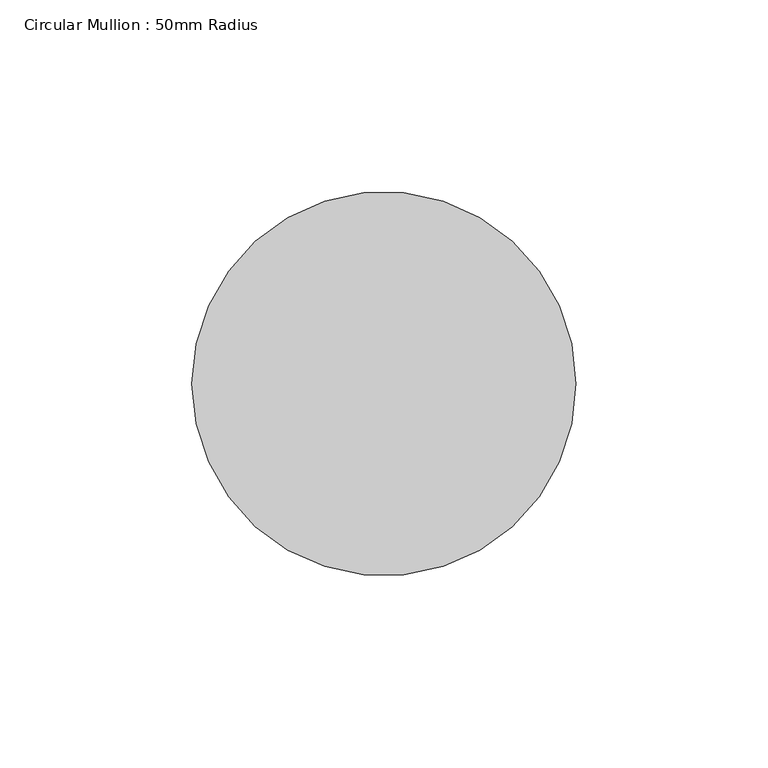
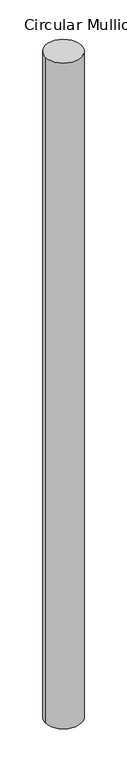
"""IFC4 building model written with IfcOpenShell, lengths in millimetres: member geometry, Circular Mullion : 50mm Radius."""

from ifc_helpers import new_model, si_unit, point, frame, frame_2d, origin, place, context, project, spatial, circle_curve, trimmed, segment, composite_curve, outline, extrude, source, transform, mapped, element, save


def circular_mullion_50mm_radius_28fe6c2a(model_context):
    return source(origin(), model_context, "Body", "SweptSolid", [
        extrude(outline(composite_curve([segment(trimmed(circle_curve(frame_2d((-50.0, 0.0)), 50.0), [point((0.0, 0.0))], [point((-100.0, 0.0))], False, "CARTESIAN"), True, "CONTINUOUS"), segment(trimmed(circle_curve(frame_2d((-50.0, 0.0)), 50.0), [point((-100.0, 0.0))], [point((0.0, 0.0))], False, "CARTESIAN"), True, "CONTINUOUS")], self_intersect=False)), frame((0.0, 0.0, -1953.2400563), z_axis=(0.0, 0.0, 1.0), x_axis=(1.0, 0.0, 0.0)), (0.0, 0.0, 1.0), 1953.2400563),
    ])


if __name__ == "__main__":
    model = new_model("IFC4")
    model_context = context("Model", 3, world=origin())
    ifc_project = project(units=[si_unit("LENGTHUNIT", "METRE", prefix="MILLI")], contexts=[model_context])
    site = spatial("IfcSite", under=ifc_project)
    building = spatial("IfcBuilding", under=site)
    placement = place(None, origin())
    circular_mullion_50mm_radius_shape = circular_mullion_50mm_radius_28fe6c2a(model_context)
    element("IfcMember", 1, ObjectType="Circular Mullion : 50mm Radius", at=placement, inside=building, context=model_context, shape_type="MappedRepresentation", body=[
        mapped(circular_mullion_50mm_radius_shape, transform((0.0, 0.0, 0.0), x_axis=(1.0, 0.0, 0.0), y_axis=(0.0, 1.0, 0.0), z_axis=(0.0, 0.0, 1.0))),
    ])
    save(model, "model.ifc")

# Revit data of these elements
# Type "Circular Mullion : 50mm Radius"
#   built-in parameter 1007350 = 0.164042 (stored number, unit not read)
# Element 1 (IfcMember, "Circular Mullion : 50mm Radius")
#   Materials on its faces: "Aluminium"
# Materials
#   "Aluminium": class "Metal", colour RGB 247 247 247, transparency 0, Description = "Aluminium 6061", Cost = 0
